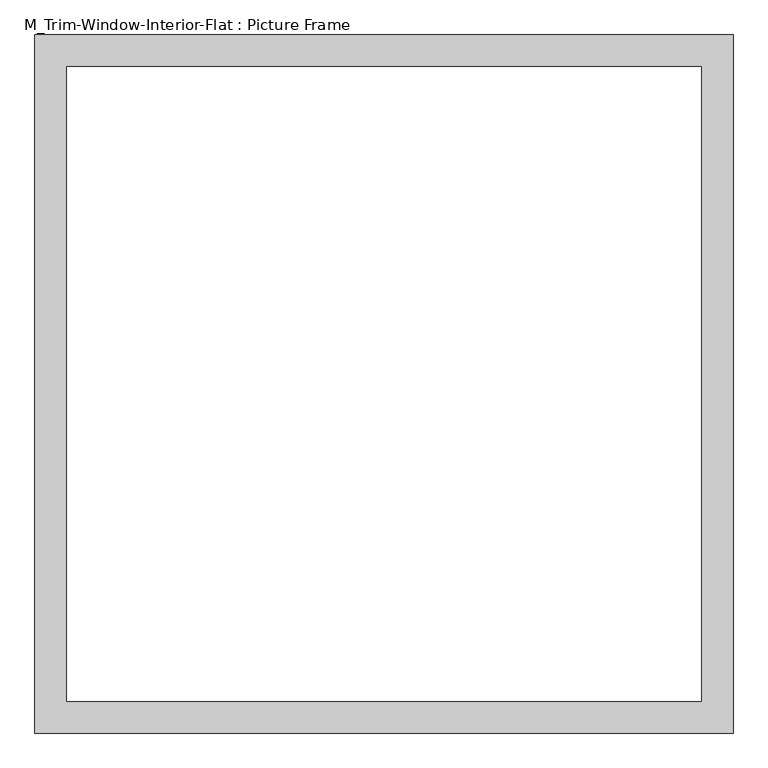
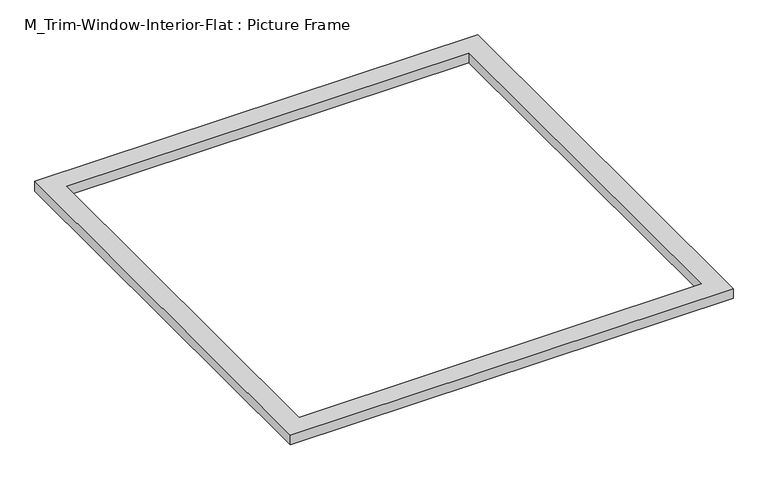
"""IFC4 building model written with IfcOpenShell, lengths in millimetres: proxy geometry, M_Trim-Window-Interior-Flat : Picture Frame."""

from ifc_helpers import new_model, si_unit, origin, origin_with_axes, place, context, project, spatial, polyline, outline, extrude, source, transform, mapped, element, save


def m_trim_window_interior_flat_picture_frame_3cf59136(model_context):
    return source(origin(), model_context, "Body", "SweptSolid", [
        extrude(outline(polyline([(656.9, -47.3), (-656.9, -47.3), (-656.9, 1266.5), (656.9, 1266.5), (656.9, -47.3)]), holes=[polyline([(596.9, 12.7), (596.9, 1206.5), (-596.9, 1206.5), (-596.9, 12.7), (596.9, 12.7)])]), origin_with_axes(), (0.0, 0.0, 1.0), 30.0),
    ])


if __name__ == "__main__":
    model = new_model("IFC4")
    model_context = context("Model", 3, world=origin())
    ifc_project = project(units=[si_unit("LENGTHUNIT", "METRE", prefix="MILLI")], contexts=[model_context])
    site = spatial("IfcSite", under=ifc_project)
    building = spatial("IfcBuilding", under=site)
    placement = place(None, origin())
    m_trim_window_interior_flat_picture_frame_shape = m_trim_window_interior_flat_picture_frame_3cf59136(model_context)
    element("IfcBuildingElementProxy", 1, Name="M_Trim-Window-Interior-Flat : Picture Frame", ObjectType="M_Trim-Window-Interior-Flat : Picture Frame", at=placement, inside=building, context=model_context, shape_type="MappedRepresentation", body=[
        mapped(m_trim_window_interior_flat_picture_frame_shape, transform((0.0, 0.0, 0.0), x_axis=(1.0, 0.0, 0.0), y_axis=(0.0, 1.0, 0.0), z_axis=(0.0, 0.0, 1.0))),
    ])
    save(model, "model.ifc")

# Revit data of these elements
# Type "M_Trim-Window-Interior-Flat : Picture Frame"
#   Trim Thickness_Picture Frame = 0' - 1.1811"
#   Trim Width = 0' - 2.3622"
#   Trim Thickness_with Sill = 0' - 0.7874"
#   Sill Thickness = 0' - 1.1811"
#   Opening Width [instance default] = 1' - 11.62205"
#   Opening Height [instance default] = 2' - 11.43307"
#   Default Elevation = 3' - 11.24409"
#   Sill = no
#   Picture Frame = yes
#   Trim Material [instance default] = none
# Element 1 (IfcBuildingElementProxy, "M_Trim-Window-Interior-Flat : Picture Frame")
#   Opening Width = 4' - 0"
#   Opening Height = 4' - 0"
#   Trim Material = Wood - Stained
#   Materials on its faces: "Wood - Stained"
# Materials
#   "Wood - Stained": class "Wood", colour RGB 224 178 126, transparency 0, Cost = 0
